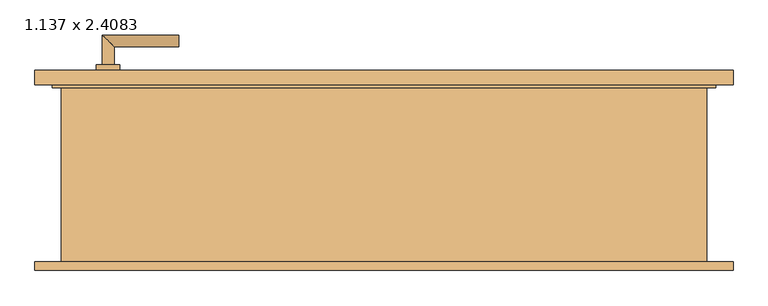
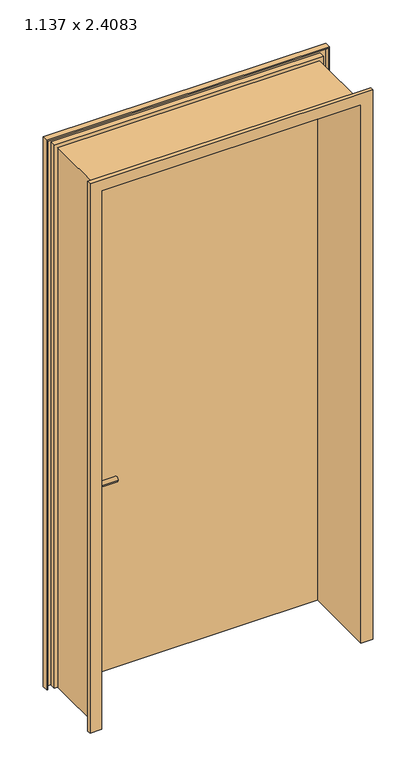
"""IFC4 building model written with IfcOpenShell, lengths in millimetres: door geometry, Drehflügel 1-flg - Stahlzarge : 1.137 x 2.4083."""

from ifc_helpers import new_model, si_unit, point, frame, frame_2d, origin, place, context, project, spatial, polyline, circle_curve, ellipse_curve, trimmed, segment, composite_curve, outline, extrude, faceted_brep, source, transform, mapped, element, save
from ifc_brep_helpers import plane_surface, cylinder_surface, advanced_brep


def door_1_137_x_2_4083_873f2a3c(model_context):
    return source(origin(), model_context, "Body", "SolidModel", [
        advanced_brep(
        [(-478.5, 139.4346141, 915.0), (-458.5, 139.4346141, 915.0), (-478.5, 69.4346141, 915.0), (-458.5, 89.4346141, 915.0), (-348.5, 69.4346141, 915.0), (-348.5, 89.4346141, 915.0)],
        [
            (0, 1, circle_curve(frame((-468.5, 139.4346141, 915.0), z_axis=(0.0, 1.0, 0.0), x_axis=(1.0, 0.0, 0.0)), 10.0)),
            (1, 0, circle_curve(frame((-468.5, 139.4346141, 915.0), z_axis=(0.0, 1.0, 0.0), x_axis=(1.0, 0.0, 0.0)), 10.0)),
            (0, 2),
            (2, 3, ellipse_curve(frame((-468.5, 79.4346141, 915.0), z_axis=(-0.7071067811865385, 0.7071067811865565, 0.0), x_axis=(0.7071067811865563, 0.7071067811865386, 0.0)), 14.1421356, 10.0)),
            (3, 1),
            (3, 2, ellipse_curve(frame((-468.5, 79.4346141, 915.0), z_axis=(-0.7071067811865385, 0.7071067811865565, 0.0), x_axis=(0.7071067811865563, 0.7071067811865386, 0.0)), 14.1421356, 10.0)),
            (4, 5, circle_curve(frame((-348.5, 79.4346141, 915.0), z_axis=(1.0, 0.0, 0.0), x_axis=(0.0, 1.0, 0.0)), 10.0)),
            (5, 4, circle_curve(frame((-348.5, 79.4346141, 915.0), z_axis=(1.0, 0.0, 0.0), x_axis=(0.0, 1.0, 0.0)), 10.0)),
            (2, 4),
            (5, 3),
        ],
        [
            plane_surface(frame((-468.5, 139.4346141, -372.7526403), z_axis=(0.0, 1.0, 0.0), x_axis=(0.0, 0.0, 1.0))),
            cylinder_surface(frame((-468.5, 139.4346141, 915.0), z_axis=(0.0, 1.0, 0.0), x_axis=(1.0, 0.0, 0.0)), 10.0),
            plane_surface(frame((-348.5, 79.4346141, -372.7526403), z_axis=(1.0, 0.0, 0.0), x_axis=(0.0, 0.0, 1.0))),
            cylinder_surface(frame((-468.5, 79.4346141, 915.0), z_axis=(-1.0, 0.0, 0.0), x_axis=(0.0, 1.0, 0.0)), 10.0),
        ],
        [
            (0, [[1, 2]]),
            (1, [[-1, 3, 4, 5]]),
            (1, [[-2, -5, 6, -3]]),
            (2, [[7, 8]]),
            (3, [[-4, 9, -8, 10]]),
            (3, [[-6, -10, -7, -9]]),
        ],
    ),
        advanced_brep(
        [(-458.5, 199.4346141, 915.0), (-478.5, 199.4346141, 915.0), (-458.5, 229.4346141, 915.0), (-478.5, 249.4346141, 915.0), (-348.5, 229.4346141, 915.0), (-348.5, 249.4346141, 915.0)],
        [
            (0, 1, circle_curve(frame((-468.5, 199.4346141, 915.0), z_axis=(0.0, -1.0, 0.0), x_axis=(-1.0, 0.0, 0.0)), 10.0)),
            (1, 0, circle_curve(frame((-468.5, 199.4346141, 915.0), z_axis=(0.0, -1.0, 0.0), x_axis=(-1.0, 0.0, 0.0)), 10.0)),
            (0, 2),
            (2, 3, ellipse_curve(frame((-468.5, 239.4346141, 915.0), z_axis=(-0.7071067811865475, -0.7071067811865475, 0.0), x_axis=(0.7071067811865474, -0.7071067811865476, 0.0)), 14.1421356, 10.0)),
            (3, 1),
            (3, 2, ellipse_curve(frame((-468.5, 239.4346141, 915.0), z_axis=(-0.7071067811865475, -0.7071067811865475, 0.0), x_axis=(0.7071067811865474, -0.7071067811865476, 0.0)), 14.1421356, 10.0)),
            (4, 5, circle_curve(frame((-348.5, 239.4346141, 915.0), z_axis=(1.0, 0.0, 0.0), x_axis=(0.0, 1.0, 0.0)), 10.0)),
            (5, 4, circle_curve(frame((-348.5, 239.4346141, 915.0), z_axis=(1.0, 0.0, 0.0), x_axis=(0.0, 1.0, 0.0)), 10.0)),
            (2, 4),
            (5, 3),
        ],
        [
            plane_surface(frame((-468.5, 199.4346141, -372.7526403), z_axis=(0.0, -1.0, 0.0), x_axis=(0.0, 0.0, 1.0))),
            cylinder_surface(frame((-468.5, 199.4346141, 915.0), z_axis=(0.0, -1.0, 0.0), x_axis=(-1.0, 0.0, 0.0)), 10.0),
            plane_surface(frame((-348.5, 239.4346141, -372.7526403), z_axis=(1.0, 0.0, 0.0), x_axis=(0.0, 0.0, 1.0))),
            cylinder_surface(frame((-468.5, 239.4346141, 915.0), z_axis=(-1.0, 0.0, 0.0), x_axis=(0.0, 1.0, 0.0)), 10.0),
        ],
        [
            (0, [[1, 2]]),
            (1, [[-1, 3, 4, 5]]),
            (1, [[-2, -5, 6, -3]]),
            (2, [[7, 8]]),
            (3, [[-4, 9, -8, 10]]),
            (3, [[-6, -10, -7, -9]]),
        ],
    ),
        extrude(outline(composite_curve([segment(trimmed(circle_curve(frame_2d((915.0, -468.5)), 20.0), [point((915.0, -488.5))], [point((915.0, -448.5))], False, "CARTESIAN"), True, "CONTINUOUS"), segment(trimmed(circle_curve(frame_2d((915.0, -468.5)), 20.0), [point((915.0, -448.5))], [point((915.0, -488.5))], False, "CARTESIAN"), True, "CONTINUOUS")], self_intersect=False)), frame((0.0, 129.4346141, 0.0), z_axis=(0.0, 1.0, 0.0), x_axis=(0.0, 0.0, 1.0)), (0.0, 0.0, 1.0), 10.0),
        extrude(outline(composite_curve([segment(trimmed(circle_curve(frame_2d((915.0, -468.5)), 20.0), [point((915.0, -488.5))], [point((915.0, -448.5))], False, "CARTESIAN"), True, "CONTINUOUS"), segment(trimmed(circle_curve(frame_2d((915.0, -468.5)), 20.0), [point((915.0, -448.5))], [point((915.0, -488.5))], False, "CARTESIAN"), True, "CONTINUOUS")], self_intersect=False)), frame((0.0, 189.4346141, 0.0), z_axis=(0.0, 1.0, 0.0), x_axis=(0.0, 0.0, 1.0)), (0.0, 0.0, 1.0), 10.0),
        extrude(outline(polyline([(558.5, 164.4346141), (-558.5, 164.4346141), (-558.5, 189.4346141), (558.5, 189.4346141), (558.5, 164.4346141)])), frame((0.0, 0.0, 15.0), z_axis=(0.0, 0.0, 1.0), x_axis=(1.0, 0.0, 0.0)), (0.0, 0.0, 1.0), 2398.3),
        faceted_brep([(592.9603207, -150.5653859, 15.0), (543.5, -150.5653859, 15.0), (543.5, 164.4346141, 15.0), (558.5, 164.4346141, 15.0), (558.5, 189.4346141, 15.0), (592.9603207, 189.4346141, 15.0), (592.9603207, 164.4346141, 15.0), (587.9603207, 164.4346141, 15.0), (587.9603207, 184.4346141, 15.0), (563.5, 184.4346141, 15.0), (563.5, 159.4346141, 15.0), (548.5, 159.4346141, 15.0), (548.5, -145.5653859, 15.0), (587.9603207, -145.5653859, 15.0), (587.9603207, -135.5653859, 15.0), (592.9603207, -135.5653859, 15.0), (592.9603207, -150.5653859, 2447.7603207), (-592.9603207, -150.5653859, 2447.7603207), (-592.9603207, -150.5653859, 15.0), (-543.5, -150.5653859, 15.0), (-543.5, -150.5653859, 2398.3), (543.5, -150.5653859, 2398.3), (543.5, 164.4346141, 2398.3), (-543.5, 164.4346141, 2398.3), (-543.5, 164.4346141, 15.0), (-558.5, 164.4346141, 15.0), (-558.5, 164.4346141, 2413.3), (558.5, 164.4346141, 2413.3), (558.5, 189.4346141, 2413.3), (-558.5, 189.4346141, 2413.3), (-558.5, 189.4346141, 15.0), (-592.9603207, 189.4346141, 15.0), (-592.9603207, 189.4346141, 2447.7603207), (592.9603207, 189.4346141, 2447.7603207), (592.9603207, 164.4346141, 2447.7603207), (-592.9603207, 164.4346141, 2447.7603207), (-592.9603207, 164.4346141, 15.0), (-587.9603207, 164.4346141, 15.0), (-587.9603207, 164.4346141, 2442.7603207), (587.9603207, 164.4346141, 2442.7603207), (587.9603207, 184.4346141, 2442.7603207), (-587.9603207, 184.4346141, 2442.7603207), (-587.9603207, 184.4346141, 15.0), (-563.5, 184.4346141, 15.0), (-563.5, 184.4346141, 2418.3), (563.5, 184.4346141, 2418.3), (563.5, 159.4346141, 2418.3), (-563.5, 159.4346141, 2418.3), (-563.5, 159.4346141, 15.0), (-548.5, 159.4346141, 15.0), (-548.5, 159.4346141, 2403.3), (548.5, 159.4346141, 2403.3), (548.5, -145.5653859, 2403.3), (-548.5, -145.5653859, 2403.3), (-548.5, -145.5653859, 15.0), (-587.9603207, -145.5653859, 15.0), (-587.9603207, -145.5653859, 2442.7603207), (587.9603207, -145.5653859, 2442.7603207), (587.9603207, -135.5653859, 2442.7603207), (-587.9603207, -135.5653859, 2442.7603207), (-587.9603207, -135.5653859, 15.0), (-592.9603207, -135.5653859, 15.0), (-592.9603207, -135.5653859, 2447.7603207), (592.9603207, -135.5653859, 2447.7603207)], [[[0, 1, 2, 3, 4, 5, 6, 7, 8, 9, 10, 11, 12, 13, 14, 15]], [[1, 0, 16, 17, 18, 19, 20, 21]], [[2, 1, 21, 22]], [[3, 2, 22, 23, 24, 25, 26, 27]], [[4, 3, 27, 28]], [[5, 4, 28, 29, 30, 31, 32, 33]], [[6, 5, 33, 34]], [[7, 6, 34, 35, 36, 37, 38, 39]], [[8, 7, 39, 40]], [[9, 8, 40, 41, 42, 43, 44, 45]], [[10, 9, 45, 46]], [[11, 10, 46, 47, 48, 49, 50, 51]], [[12, 11, 51, 52]], [[13, 12, 52, 53, 54, 55, 56, 57]], [[14, 13, 57, 58]], [[15, 14, 58, 59, 60, 61, 62, 63]], [[0, 15, 63, 16]], [[17, 62, 61, 18]], [[18, 61, 60, 55, 54, 49, 48, 43, 42, 37, 36, 31, 30, 25, 24, 19]], [[23, 20, 19, 24]], [[29, 26, 25, 30]], [[35, 32, 31, 36]], [[41, 38, 37, 42]], [[47, 44, 43, 48]], [[53, 50, 49, 54]], [[59, 56, 55, 60]], [[22, 21, 20, 23]], [[28, 27, 26, 29]], [[34, 33, 32, 35]], [[40, 39, 38, 41]], [[46, 45, 44, 47]], [[52, 51, 50, 53]], [[58, 57, 56, 59]], [[16, 63, 62, 17]]]),
    ])


if __name__ == "__main__":
    model = new_model("IFC4")
    model_context = context("Model", 3, world=origin())
    ifc_project = project(units=[si_unit("LENGTHUNIT", "METRE", prefix="MILLI")], contexts=[model_context])
    site = spatial("IfcSite", under=ifc_project)
    building = spatial("IfcBuilding", under=site)
    placement = place(None, origin())
    door_1_137_x_2_4083_shape = door_1_137_x_2_4083_873f2a3c(model_context)
    element("IfcDoor", 1, ObjectType="Drehflügel 1-flg - Stahlzarge : 1.137 x 2.4083", at=placement, inside=building, context=model_context, shape_type="MappedRepresentation", body=[
        mapped(door_1_137_x_2_4083_shape, transform((0.0, 0.0, 0.0), x_axis=(1.0, 0.0, 0.0), y_axis=(0.0, 1.0, 0.0), z_axis=(0.0, 0.0, 1.0))),
    ])
    save(model, "model.ifc")

# Revit data of these elements
# Type "Drehflügel 1-flg - Stahlzarge : 1.137 x 2.4083"
#   Type Mark = "21"
#   Operation = "SingleSwingRight"
#   Keynote = "16.03"
#   Analytic Construction = "Metall"
#   Thermal Resistance (R) = 0.270117 (m²·K)/W
#   Heat Transfer Coefficient (U) = 3.7021 W/(m²·K)
#   Rough Width = 1.137 m
#   Rough Height [instance default] = 2.5083 m
#   Höhe Türgriff [instance default] = 0.900 m
#   Height = 2.4083 m
#   Fußbodenaufbau [instance default] = 0.100 m
#   Width = 1.137 m
#   Sichtbarkeit Sturzlinien [instance default] = yes
#   Türgriff auswählen [instance default] = element 221079
#   Türgriff [instance default] = none
#   Türflügel [instance default] = none
#   Rahmen/Pfosten [instance default] = Metall - Lackiert - Grau
#   Visual Light Transmittance = 0
#   Solar Heat Gain Coefficient = 0
#   Function = (empty or 0)
#   Wall Closure = (empty or 0)
# Element 1 (IfcDoor, "Drehflügel 1-flg - Stahlzarge : 1.137 x 2.4083")
#   Rough Height = 2.4233 m
#   Fußbodenaufbau = 0.015 m
#   Materials on its faces: "Metall - Lackiert - Grau", "Metall - Chrom", "Holz - Birke"
# Materials
#   "Metall - Lackiert - Grau": class "Farbe 1", colour RGB 98 98 98, transparency 0, Cost = 0
#   "Metall - Chrom": class "Metall", colour RGB 247 247 247, transparency 0, Cost = 0
#   "Holz - Birke": class "Holz", colour RGB 213 164 103, transparency 0, Cost = 0
